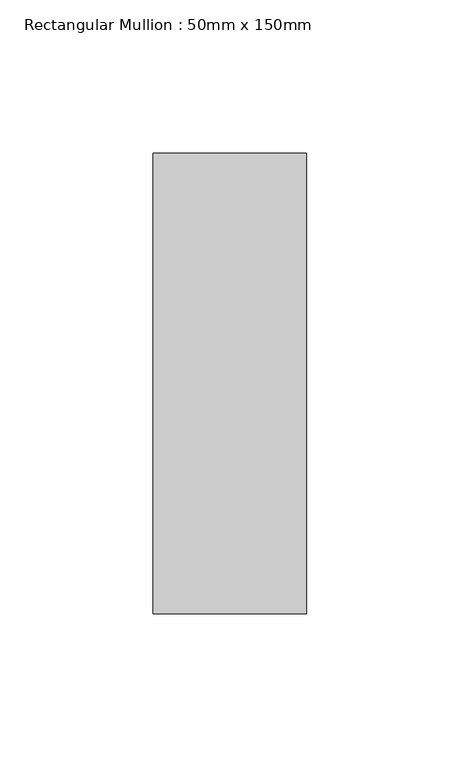
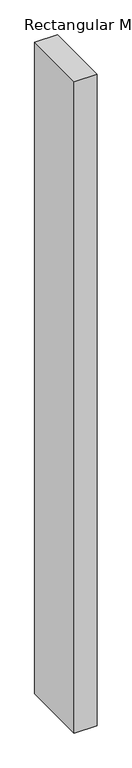
"""IFC4 building model written with IfcOpenShell, lengths in millimetres: member geometry, Rectangular Mullion : 50mm x 150mm."""

from ifc_helpers import new_model, si_unit, frame, origin, place, context, project, spatial, polyline, outline, extrude, source, transform, mapped, element, save


def rectangular_mullion_50mm_x_150mm_86585c2a(model_context):
    return source(origin(), model_context, "Body", "SweptSolid", [
        extrude(outline(polyline([(0.0, 75.0), (0.0, -75.0), (-50.0, -75.0), (-50.0, 75.0), (0.0, 75.0)])), frame((0.0, 0.0, -1511.0169252), z_axis=(0.0, 0.0, 1.0), x_axis=(1.0, 0.0, 0.0)), (0.0, 0.0, 1.0), 1511.0169252),
    ])


if __name__ == "__main__":
    model = new_model("IFC4")
    model_context = context("Model", 3, world=origin())
    ifc_project = project(units=[si_unit("LENGTHUNIT", "METRE", prefix="MILLI")], contexts=[model_context])
    site = spatial("IfcSite", under=ifc_project)
    building = spatial("IfcBuilding", under=site)
    placement = place(None, origin())
    rectangular_mullion_50mm_x_150mm_shape = rectangular_mullion_50mm_x_150mm_86585c2a(model_context)
    element("IfcMember", 1, ObjectType="Rectangular Mullion : 50mm x 150mm", at=placement, inside=building, context=model_context, shape_type="MappedRepresentation", body=[
        mapped(rectangular_mullion_50mm_x_150mm_shape, transform((0.0, 0.0, 0.0), x_axis=(1.0, 0.0, 0.0), y_axis=(0.0, 1.0, 0.0), z_axis=(0.0, 0.0, 1.0))),
    ])
    save(model, "model.ifc")

# Revit data of these elements
# Type "Rectangular Mullion : 50mm x 150mm"
#   built-in parameter 1007304 = 0.492126 (stored number, unit not read)
#   built-in parameter 1007301 = 0.082021 (stored number, unit not read)
#   built-in parameter 1007300 = 0.082021 (stored number, unit not read)
# Element 1 (IfcMember, "Rectangular Mullion : 50mm x 150mm")
#   Materials on its faces: "Aluminum"
# Materials
#   "Aluminum": class "Metal", colour RGB 244 244 244, transparency 0, Description = "Aluminum 6061", Cost = 0
